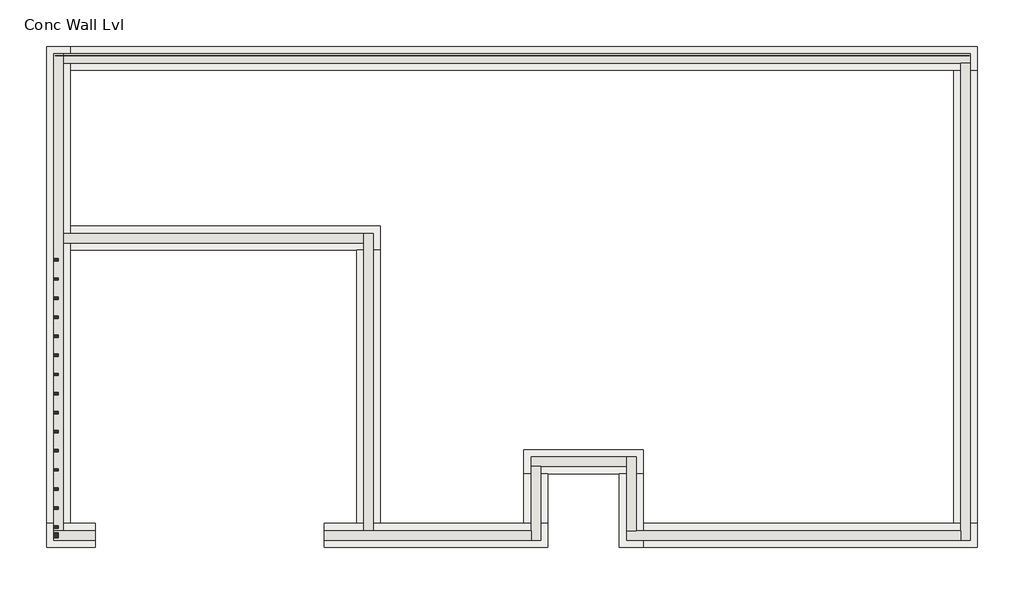
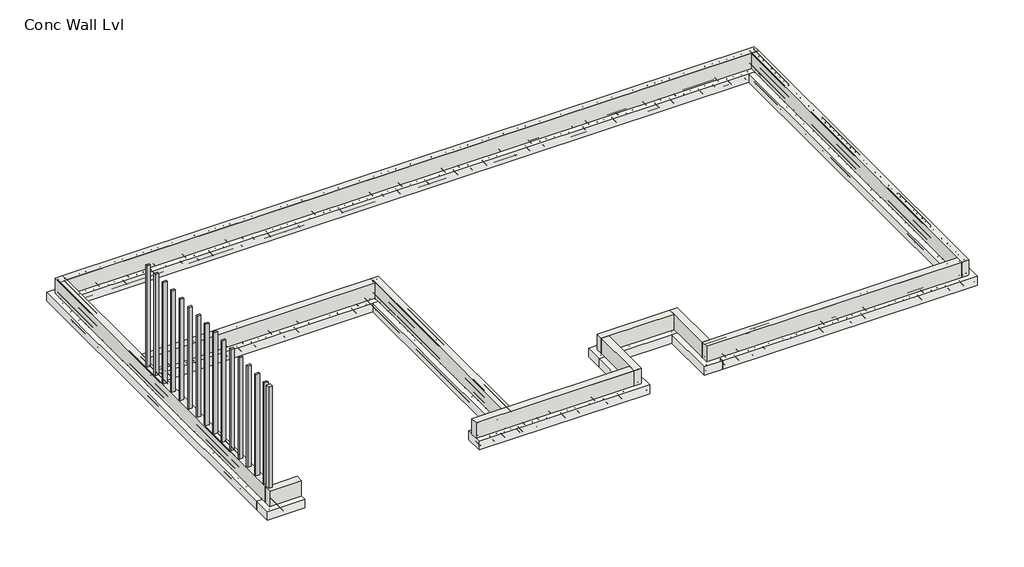
# One storey, part 1 of 4: 16 columns, 11 footings, 11 walls.
"""IFC4 building model written with IfcOpenShell, lengths in millimetres."""

import ifcopenshell
import ifcopenshell.guid

model = None  # the IFC model being written
_history = None  # IfcOwnerHistory: only IFC2X3 demands one
_inside = {}  # id of a spatial element -> (the spatial element, [elements in it])
_under = {}  # id of a project, library or spatial element -> (it, [spatial elements below it])
_declared = {}  # id of a project -> (the project, [libraries it declares])
_typed = {}  # id of a type object -> (the type object, [elements of that type])
_made_of = {}  # id of a material, layer set ... -> (it, [elements and type objects made of it])


def new_model(schema):
    """Start an empty IFC model of exactly this schema.

    Asked for "IFC4X3", IfcOpenShell would pick the latest addendum, in which some entities
    have other attributes; the version numbers below select the first issue.
    IFC2X3 requires an IfcOwnerHistory on every rooted entity: one is made here for all.
    """
    global model, _history
    if schema == "IFC4X3":
        model = ifcopenshell.file(schema_version=(4, 3, 0, 0))
    else:
        model = ifcopenshell.file(schema=schema)
    _inside.clear()
    _under.clear()
    _declared.clear()
    _typed.clear()
    _made_of.clear()
    _history = None
    if model.schema == "IFC2X3":
        org = make("IfcOrganization", Name="unknown")
        user = make(
            "IfcPersonAndOrganization",
            ThePerson=make("IfcPerson", FamilyName="unknown"),
            TheOrganization=org,
        )
        app = make(
            "IfcApplication",
            ApplicationDeveloper=org,
            Version="unknown",
            ApplicationFullName="unknown",
            ApplicationIdentifier="unknown",
        )
        _history = make(
            "IfcOwnerHistory",
            OwningUser=user,
            OwningApplication=app,
            ChangeAction="ADDED",
            CreationDate=0,
        )
    return model


def make(cls, **values):
    """One entity of the class cls with the attributes given. An attribute that is None is left unset."""
    return model.create_entity(
        cls, **{name: value for name, value in values.items() if value is not None}
    )


def rooted(cls, **values):
    """An entity with a GlobalId (a new one), such as an element, a storey or a relation."""
    return make(cls, GlobalId=ifcopenshell.guid.new(), OwnerHistory=_history, **values)


def si_unit(unit_type, name, prefix=None):
    """IfcSIUnit, for example si_unit("LENGTHUNIT", "METRE", prefix="MILLI")."""
    return make("IfcSIUnit", UnitType=unit_type, Prefix=prefix, Name=name)


def assignment(units):
    """IfcUnitAssignment: the units of a project."""
    return None if units is None else make("IfcUnitAssignment", Units=units)


def point(xyz):
    """IfcCartesianPoint."""
    return None if xyz is None else make("IfcCartesianPoint", Coordinates=xyz)


def direction(xyz):
    """IfcDirection."""
    return None if xyz is None else make("IfcDirection", DirectionRatios=xyz)


def frame(location, z_axis=None, x_axis=None):
    """IfcAxis2Placement3D, a coordinate frame: its origin and axes. An axis left out is left unset."""
    return make(
        "IfcAxis2Placement3D",
        Location=point(location),
        Axis=direction(z_axis),
        RefDirection=direction(x_axis),
    )


def origin():
    """The frame at (0, 0, 0) with its axes left unset."""
    return frame((0.0, 0.0, 0.0))


def place(relative_to, where):
    """IfcLocalPlacement: puts the frame where relative to a parent placement (None: the world)."""
    return make(
        "IfcLocalPlacement", PlacementRelTo=relative_to, RelativePlacement=where
    )


def context(
    kind, dimensions, precision=None, world=None, true_north=None, identifier=None
):
    """IfcGeometricRepresentationContext, for example the 3D "Model" context."""
    return make(
        "IfcGeometricRepresentationContext",
        ContextIdentifier=identifier,
        ContextType=kind,
        CoordinateSpaceDimension=dimensions,
        Precision=precision,
        WorldCoordinateSystem=world,
        TrueNorth=true_north,
    )


def project(units=None, contexts=None):
    """IfcProject with its units and contexts."""
    return rooted(
        "IfcProject",
        Name="project",
        RepresentationContexts=contexts,
        UnitsInContext=assignment(units),
    )


def spatial(cls, under=None, at=None, **own):
    """A site, building, storey or space (cls), placed at a placement, below another one or the project."""
    s = rooted(cls, ObjectPlacement=at, **own)
    if under is not None:
        _under.setdefault(under.id(), (under, []))[1].append(s)
    return s


def polyline(points):
    """IfcPolyline through the points."""
    return make("IfcPolyline", Points=[point(p) for p in points])


def outline(outer, holes=None, kind="AREA"):
    """IfcArbitraryClosedProfileDef: a profile drawn as a closed curve; with holes, ...WithVoids."""
    if holes is None:
        return make("IfcArbitraryClosedProfileDef", ProfileType=kind, OuterCurve=outer)
    return make(
        "IfcArbitraryProfileDefWithVoids",
        ProfileType=kind,
        OuterCurve=outer,
        InnerCurves=holes,
    )


def extrude(swept, where, along, depth):
    """IfcExtrudedAreaSolid: the profile swept, set in the frame where, extruded along a direction by depth."""
    return make(
        "IfcExtrudedAreaSolid",
        SweptArea=swept,
        Position=where,
        ExtrudedDirection=direction(along),
        Depth=depth,
    )


def faces_of(points, faces, orient=None, outer=None):
    """IfcFace entities. A face is a list of loops; a loop is a list of indices into points, from 0.

    orient and outer hold one flag for each loop. By default every Orientation is true, the
    first loop of a face is its IfcFaceOuterBound and the others are IfcFaceBound.
    """
    made = []
    for i, loops in enumerate(faces):
        bounds = []
        for j, loop in enumerate(loops):
            is_outer = j == 0 if outer is None else outer[i][j]
            bounds.append(
                make(
                    "IfcFaceOuterBound" if is_outer else "IfcFaceBound",
                    Bound=make("IfcPolyLoop", Polygon=[points[k] for k in loop]),
                    Orientation=True if orient is None else orient[i][j],
                )
            )
        made.append(make("IfcFace", Bounds=bounds))
    return made


def faceted_brep(points, faces, orient=None, outer=None, voids=None):
    """IfcFacetedBrep: a solid bounded by flat faces; with voids (closed shells), ...WithVoids."""
    shared = [point(p) for p in points]
    hull = make("IfcClosedShell", CfsFaces=faces_of(shared, faces, orient, outer))
    if voids is None:
        return make("IfcFacetedBrep", Outer=hull)
    return make(
        "IfcFacetedBrepWithVoids",
        Outer=hull,
        Voids=[
            make(cls, CfsFaces=faces_of(shared, fs, o, b)) for cls, fs, o, b in voids
        ],
    )


def shape(context_of_items, identifier, shape_type, items):
    """IfcShapeRepresentation: the items that make up one representation, for example the "Body"."""
    return make(
        "IfcShapeRepresentation",
        ContextOfItems=context_of_items,
        RepresentationIdentifier=identifier,
        RepresentationType=shape_type,
        Items=items,
    )


def source(mapping_origin, context_of_items, identifier, shape_type, items):
    """IfcRepresentationMap: a shape defined once, which mapped items show again and again."""
    return make(
        "IfcRepresentationMap",
        MappingOrigin=mapping_origin,
        MappedRepresentation=shape(context_of_items, identifier, shape_type, items),
    )


def transform(
    local_origin,
    x_axis=None,
    y_axis=None,
    z_axis=None,
    scale=None,
    scale2=None,
    scale3=None,
    uniform=True,
):
    """IfcCartesianTransformationOperator3D, or its non-uniform kind. x_axis, y_axis, z_axis: its Axis1, 2, 3."""
    if uniform:
        return make(
            "IfcCartesianTransformationOperator3D",
            Axis1=direction(x_axis),
            Axis2=direction(y_axis),
            LocalOrigin=point(local_origin),
            Scale=scale,
            Axis3=direction(z_axis),
        )
    return make(
        "IfcCartesianTransformationOperator3DnonUniform",
        Axis1=direction(x_axis),
        Axis2=direction(y_axis),
        LocalOrigin=point(local_origin),
        Scale=scale,
        Axis3=direction(z_axis),
        Scale2=scale2,
        Scale3=scale3,
    )


def mapped(mapping_source, mapping_target):
    """IfcMappedItem: shows the shape of a source again, moved by a transform."""
    return make(
        "IfcMappedItem", MappingSource=mapping_source, MappingTarget=mapping_target
    )


def made_of(thing, what):
    """Note that an element or type object is made of a material, layer set ...; save() writes the relation."""
    if what is not None:
        _made_of.setdefault(what.id(), (what, []))[1].append(thing)
    return thing


def element(
    cls,
    number,
    at=None,
    inside=None,
    cuts=None,
    type_object=None,
    material=None,
    context=None,
    identifier="Body",
    shape_type=None,
    held_by="IfcProductDefinitionShape",
    body=None,
    shapes=None,
    **own,
):
    """One element of the class cls, such as IfcWall. Its Tag is "e" and its number.

    at: its placement. inside: the storey or other place that contains it. cuts: it is an
    opening in that element (IfcRelVoidsElement). A single representation is given by context,
    identifier, shape_type and body (its items); several are given by shapes. held_by: the class
    of the entity that holds the representations. save() writes the other relations.
    """
    e = rooted(cls, Tag="e%d" % number, ObjectPlacement=at, **own)
    if body is not None:
        shapes = [shape(context, identifier, shape_type, body)]
    if shapes is not None:
        e.Representation = make(held_by, Representations=shapes)
    if inside is not None:
        _inside.setdefault(inside.id(), (inside, []))[1].append(e)
    if cuts is not None:
        rooted(
            "IfcRelVoidsElement", RelatingBuildingElement=cuts, RelatedOpeningElement=e
        )
    if type_object is not None:
        _typed.setdefault(type_object.id(), (type_object, []))[1].append(e)
    return made_of(e, material)


def aggregate(whole, parts):
    """IfcRelAggregates: a whole, such as a stair, and the parts it consists of."""
    return rooted("IfcRelAggregates", RelatingObject=whole, RelatedObjects=parts)


def save(model, path):
    """Write the relations noted so far, then the file.

    IfcRelAggregates (storeys below a building ...), IfcRelContainedInSpatialStructure (elements
    in a storey), IfcRelDefinesByType, IfcRelAssociatesMaterial and IfcRelDeclares: one each for
    every whole, place, type object, material and project.
    """
    for whole, parts in _under.values():
        aggregate(whole, parts)
    for where, things in _inside.values():
        rooted(
            "IfcRelContainedInSpatialStructure",
            RelatedElements=things,
            RelatingStructure=where,
        )
    for kind, things in _typed.values():
        rooted("IfcRelDefinesByType", RelatedObjects=things, RelatingType=kind)
    for what, things in _made_of.values():
        rooted("IfcRelAssociatesMaterial", RelatedObjects=things, RelatingMaterial=what)
    for by, libraries in _declared.values():
        rooted("IfcRelDeclares", RelatingContext=by, RelatedDefinitions=libraries)
    model.write(path)


def timber_column_4ee0a357(model_context):
    return source(origin(), model_context, "Body", "SweptSolid", [
        extrude(outline(polyline([(25.4, 50.8), (25.4, -50.8), (-25.4, -50.8), (-25.4, 50.8), (25.4, 50.8)])), frame((0.0, 0.0, -319.88125), z_axis=(0.0, 0.0, 1.0), x_axis=(1.0, 0.0, 0.0)), (0.0, 0.0, 1.0), 2986.88125),
    ])


def timber_column_8a3ad47c(model_context):
    return source(origin(), model_context, "Body", "SweptSolid", [
        extrude(outline(polyline([(50.8, 50.8), (50.8, -50.8), (-50.8, -50.8), (-50.8, 50.8), (50.8, 50.8)])), frame((0.0, 0.0, -319.88125), z_axis=(0.0, 0.0, 1.0), x_axis=(1.0, 0.0, 0.0)), (0.0, 0.0, 1.0), 2986.88125),
    ])


model = new_model("IFC4")

# Units and contexts
model_context = context("Model", 3, world=origin())
ifc_project = project(units=[si_unit("LENGTHUNIT", "METRE", prefix="MILLI")], contexts=[model_context])

# Site, building, storey
site = spatial("IfcSite", under=ifc_project)
building = spatial("IfcBuilding", under=site)
storey = spatial("IfcBuildingStorey", under=building, Name="Conc Wall Lvl", Elevation=-370.68125)

# Columns
placement = place(None, origin())
timber_column_shape = timber_column_4ee0a357(model_context)
element("IfcColumn", 1, ObjectType="Timber-Column : BLDG 6241 Wall Struds 2\"x4\"", at=placement, inside=storey, context=model_context, shape_type="MappedRepresentation", body=[
    mapped(timber_column_shape, transform((-17750.414829, 813.5284114, 0.0), x_axis=(0.0, 1.0, 0.0), y_axis=(-1.0, 0.0, 0.0), z_axis=(0.0, 0.0, 1.0))),
])
element("IfcColumn", 2, ObjectType="Timber-Column : BLDG 6241 Wall Struds 2\"x4\"", at=placement, inside=storey, context=model_context, shape_type="MappedRepresentation", body=[
    mapped(timber_column_shape, transform((-17750.414829, 407.1284114, 0.0), x_axis=(0.0, 1.0, 0.0), y_axis=(-1.0, 0.0, 0.0), z_axis=(0.0, 0.0, 1.0))),
])
element("IfcColumn", 3, ObjectType="Timber-Column : BLDG 6241 Wall Struds 2\"x4\"", at=placement, inside=storey, context=model_context, shape_type="MappedRepresentation", body=[
    mapped(timber_column_shape, transform((-17750.414829, 0.7284114, 0.0), x_axis=(0.0, 1.0, 0.0), y_axis=(-1.0, 0.0, 0.0), z_axis=(0.0, 0.0, 1.0))),
])
element("IfcColumn", 4, ObjectType="Timber-Column : BLDG 6241 Wall Struds 2\"x4\"", at=placement, inside=storey, context=model_context, shape_type="MappedRepresentation", body=[
    mapped(timber_column_shape, transform((-17750.414829, -405.6715886, 0.0), x_axis=(0.0, 1.0, 0.0), y_axis=(-1.0, 0.0, 0.0), z_axis=(0.0, 0.0, 1.0))),
])
element("IfcColumn", 5, ObjectType="Timber-Column : BLDG 6241 Wall Struds 2\"x4\"", at=placement, inside=storey, context=model_context, shape_type="MappedRepresentation", body=[
    mapped(timber_column_shape, transform((-17750.414829, -812.0715886, 0.0), x_axis=(0.0, 1.0, 0.0), y_axis=(-1.0, 0.0, 0.0), z_axis=(0.0, 0.0, 1.0))),
])
element("IfcColumn", 6, ObjectType="Timber-Column : BLDG 6241 Wall Struds 2\"x4\"", at=placement, inside=storey, context=model_context, shape_type="MappedRepresentation", body=[
    mapped(timber_column_shape, transform((-17750.414829, -1218.4715886, 0.0), x_axis=(0.0, 1.0, 0.0), y_axis=(-1.0, 0.0, 0.0), z_axis=(0.0, 0.0, 1.0))),
])
element("IfcColumn", 7, ObjectType="Timber-Column : BLDG 6241 Wall Struds 2\"x4\"", at=placement, inside=storey, context=model_context, shape_type="MappedRepresentation", body=[
    mapped(timber_column_shape, transform((-17750.414829, -1624.8715886, 0.0), x_axis=(0.0, 1.0, 0.0), y_axis=(-1.0, 0.0, 0.0), z_axis=(0.0, 0.0, 1.0))),
])
element("IfcColumn", 8, ObjectType="Timber-Column : BLDG 6241 Wall Struds 2\"x4\"", at=placement, inside=storey, context=model_context, shape_type="MappedRepresentation", body=[
    mapped(timber_column_shape, transform((-17750.414829, -2031.2715886, 0.0), x_axis=(0.0, 1.0, 0.0), y_axis=(-1.0, 0.0, 0.0), z_axis=(0.0, 0.0, 1.0))),
])
element("IfcColumn", 9, ObjectType="Timber-Column : BLDG 6241 Wall Struds 2\"x4\"", at=placement, inside=storey, context=model_context, shape_type="MappedRepresentation", body=[
    mapped(timber_column_shape, transform((-17750.414829, -2437.6715886, 0.0), x_axis=(0.0, 1.0, 0.0), y_axis=(-1.0, 0.0, 0.0), z_axis=(0.0, 0.0, 1.0))),
])
element("IfcColumn", 10, ObjectType="Timber-Column : BLDG 6241 Wall Struds 2\"x4\"", at=placement, inside=storey, context=model_context, shape_type="MappedRepresentation", body=[
    mapped(timber_column_shape, transform((-17750.414829, -2844.0715886, 0.0), x_axis=(0.0, 1.0, 0.0), y_axis=(-1.0, 0.0, 0.0), z_axis=(0.0, 0.0, 1.0))),
])
element("IfcColumn", 11, ObjectType="Timber-Column : BLDG 6241 Wall Struds 2\"x4\"", at=placement, inside=storey, context=model_context, shape_type="MappedRepresentation", body=[
    mapped(timber_column_shape, transform((-17750.414829, -3250.4715886, 0.0), x_axis=(0.0, 1.0, 0.0), y_axis=(-1.0, 0.0, 0.0), z_axis=(0.0, 0.0, 1.0))),
])
element("IfcColumn", 12, ObjectType="Timber-Column : BLDG 6241 Wall Struds 2\"x4\"", at=placement, inside=storey, context=model_context, shape_type="MappedRepresentation", body=[
    mapped(timber_column_shape, transform((-17750.414829, -3656.8715886, 0.0), x_axis=(0.0, 1.0, 0.0), y_axis=(-1.0, 0.0, 0.0), z_axis=(0.0, 0.0, 1.0))),
])
element("IfcColumn", 13, ObjectType="Timber-Column : BLDG 6241 Wall Struds 2\"x4\"", at=placement, inside=storey, context=model_context, shape_type="MappedRepresentation", body=[
    mapped(timber_column_shape, transform((-17750.414829, -4063.2715886, 0.0), x_axis=(0.0, 1.0, 0.0), y_axis=(-1.0, 0.0, 0.0), z_axis=(0.0, 0.0, 1.0))),
])
element("IfcColumn", 14, ObjectType="Timber-Column : BLDG 6241 Wall Struds 2\"x4\"", at=placement, inside=storey, context=model_context, shape_type="MappedRepresentation", body=[
    mapped(timber_column_shape, transform((-17750.414829, -4469.6715886, 0.0), x_axis=(0.0, 1.0, 0.0), y_axis=(-1.0, 0.0, 0.0), z_axis=(0.0, 0.0, 1.0))),
])
element("IfcColumn", 15, ObjectType="Timber-Column : BLDG 6241 Wall Struds 2\"x4\"", at=placement, inside=storey, context=model_context, shape_type="MappedRepresentation", body=[
    mapped(timber_column_shape, transform((-17750.414829, -4876.0715886, 0.0), x_axis=(0.0, 1.0, 0.0), y_axis=(-1.0, 0.0, 0.0), z_axis=(0.0, 0.0, 1.0))),
])
timber_column_2_shape = timber_column_8a3ad47c(model_context)
element("IfcColumn", 16, ObjectType="Timber-Column : BLDG 6241 Wall Struds 4\"x4\"", at=placement, inside=storey, context=model_context, shape_type="MappedRepresentation", body=[
    mapped(timber_column_2_shape, transform((-17750.414829, -5053.8715886, 0.0), x_axis=(1.0, 0.0, 0.0), y_axis=(0.0, 1.0, 0.0), z_axis=(0.0, 0.0, 1.0))),
])

# Footings
element("IfcFooting", 17, ObjectType="BLDG Conc Footing - 20\" x 10\"", at=placement, inside=storey, context=model_context, shape_type="Brep", body=[
    faceted_brep([(-16915.389829, -4799.8715886, -827.88125), (-16915.389829, -5307.8715886, -827.88125), (-16915.389829, -5307.8715886, -1081.88125), (-16915.389829, -4799.8715886, -1081.88125), (-17445.614829, -4799.8715886, -827.88125), (-17953.614829, -4799.8715886, -827.88125), (-17953.614829, -5307.8715886, -827.88125), (-17953.614829, -5307.8715886, -1081.88125), (-17953.614829, -4799.8715886, -1081.88125), (-17445.614829, -4799.8715886, -1081.88125)], [[[0, 1, 2, 3]], [[0, 4, 5, 6, 1]], [[2, 1, 6, 7]], [[3, 2, 7, 8, 9]], [[0, 3, 9, 8, 5, 4]], [[6, 5, 8, 7]]]),
])
element("IfcFooting", 18, ObjectType="BLDG Conc Footing - 20\" x 10\"", at=placement, inside=storey, context=model_context, shape_type="Brep", body=[
    faceted_brep([(-17445.614829, 5360.1284114, -827.88125), (-17953.614829, 5360.1284114, -827.88125), (-17953.614829, -4799.8715886, -827.88125), (-17445.614829, -4799.8715886, -827.88125), (-17445.614829, 1023.0784114, -827.88125), (-17445.614829, 1531.0784114, -827.88125), (-17445.614829, 4852.1284114, -827.88125), (-17953.614829, 5360.1284114, -1081.88125), (-17953.614829, -4799.8715886, -1081.88125), (-17445.614829, 5360.1284114, -1081.88125), (-17445.614829, 4852.1284114, -1081.88125), (-17445.614829, 1531.0784114, -1081.88125), (-17445.614829, 1023.0784114, -1081.88125), (-17445.614829, -4799.8715886, -1081.88125)], [[[0, 1, 2, 3, 4, 5, 6]], [[1, 7, 8, 2]], [[7, 9, 10, 11, 12, 13, 8]], [[9, 0, 6, 5, 4, 3, 13, 12, 11, 10]], [[3, 2, 8, 13]], [[1, 0, 9, 7]]]),
])
element("IfcFooting", 19, ObjectType="BLDG Conc Footing - 20\" x 10\"", at=placement, inside=storey, context=model_context, shape_type="Brep", body=[
    faceted_brep([(-10847.964829, 1531.0784114, -827.88125), (-17445.614829, 1531.0784114, -827.88125), (-17445.614829, 1023.0784114, -827.88125), (-11355.964829, 1023.0784114, -827.88125), (-10847.964829, 1023.0784114, -827.88125), (-10847.964829, 1023.0784114, -1081.88125), (-17445.614829, 1023.0784114, -1081.88125), (-11355.964829, 1023.0784114, -1081.88125), (-10847.964829, 1531.0784114, -1081.88125), (-17445.614829, 1531.0784114, -1081.88125)], [[[0, 1, 2, 3, 4]], [[5, 4, 3, 2, 6, 7]], [[8, 5, 7, 6, 9]], [[0, 8, 9, 1]], [[2, 1, 9, 6]], [[0, 4, 5, 8]]]),
])
element("IfcFooting", 20, ObjectType="BLDG Conc Footing - 20\" x 10\"", at=placement, inside=storey, context=model_context, shape_type="SweptSolid", body=[
    extrude(outline(polyline([(-10847.964829, -4799.8715886), (-11355.964829, -4799.8715886), (-11355.964829, 1023.0784114), (-10847.964829, 1023.0784114), (-10847.964829, -4799.8715886)])), frame((0.0, 0.0, -1081.88125), z_axis=(0.0, 0.0, 1.0), x_axis=(1.0, 0.0, 0.0)), (0.0, 0.0, 1.0), 254.0),
])
element("IfcFooting", 21, ObjectType="BLDG Conc Footing - 20\" x 10\"", at=placement, inside=storey, context=model_context, shape_type="Brep", body=[
    faceted_brep([(-12038.589829, -5307.8715886, -827.88125), (-12038.589829, -4799.8715886, -827.88125), (-12038.589829, -4799.8715886, -1081.88125), (-12038.589829, -5307.8715886, -1081.88125), (-7285.614829, -4799.8715886, -827.88125), (-7793.614829, -4799.8715886, -827.88125), (-10847.964829, -4799.8715886, -827.88125), (-11355.964829, -4799.8715886, -827.88125), (-7285.614829, -5307.8715886, -827.88125), (-7285.614829, -5307.8715886, -1081.88125), (-7285.614829, -4799.8715886, -1081.88125), (-11355.964829, -4799.8715886, -1081.88125), (-10847.964829, -4799.8715886, -1081.88125), (-7793.614829, -4799.8715886, -1081.88125)], [[[0, 1, 2, 3]], [[4, 5, 6, 7, 1, 0, 8]], [[9, 8, 0, 3]], [[10, 9, 3, 2, 11, 12, 13]], [[4, 10, 13, 12, 11, 2, 1, 7, 6, 5]], [[4, 8, 9, 10]]]),
])
element("IfcFooting", 22, ObjectType="BLDG Conc Footing - 20\" x 10\"", at=placement, inside=storey, context=model_context, shape_type="Brep", body=[
    faceted_brep([(-5253.614829, -3231.4215886, -827.88125), (-7793.614829, -3231.4215886, -827.88125), (-7793.614829, -3739.4215886, -827.88125), (-7285.614829, -3739.4215886, -827.88125), (-5761.614829, -3739.4215886, -827.88125), (-5253.614829, -3739.4215886, -827.88125), (-5253.614829, -3739.4215886, -1081.88125), (-7793.614829, -3739.4215886, -1081.88125), (-7285.614829, -3739.4215886, -1081.88125), (-5761.614829, -3739.4215886, -1081.88125), (-5253.614829, -3231.4215886, -1081.88125), (-7793.614829, -3231.4215886, -1081.88125)], [[[0, 1, 2, 3, 4, 5]], [[6, 5, 4, 3, 2, 7, 8, 9]], [[10, 6, 9, 8, 7, 11]], [[0, 10, 11, 1]], [[0, 5, 6, 10]], [[2, 1, 11, 7]]]),
])
element("IfcFooting", 23, ObjectType="BLDG Conc Footing - 20\" x 10\"", at=placement, inside=storey, context=model_context, shape_type="Brep", body=[
    faceted_brep([(-5761.614829, -5307.8715886, -827.88125), (-5253.614829, -5307.8715886, -827.88125), (-5253.614829, -4799.8715886, -827.88125), (-5253.614829, -3739.4215886, -827.88125), (-5761.614829, -3739.4215886, -827.88125), (-5761.614829, -5307.8715886, -1081.88125), (-5761.614829, -3739.4215886, -1081.88125), (-5253.614829, -5307.8715886, -1081.88125), (-5253.614829, -3739.4215886, -1081.88125), (-5253.614829, -4799.8715886, -1081.88125)], [[[0, 1, 2, 3, 4]], [[5, 0, 4, 6]], [[7, 5, 6, 8, 9]], [[1, 7, 9, 8, 3, 2]], [[4, 3, 8, 6]], [[1, 0, 5, 7]]]),
])
element("IfcFooting", 24, ObjectType="BLDG Conc Footing - 20\" x 10\"", at=placement, inside=storey, context=model_context, shape_type="Brep", body=[
    faceted_brep([(1858.385171, -5307.8715886, -827.88125), (1858.385171, -4799.8715886, -827.88125), (1350.385171, -4799.8715886, -827.88125), (-5253.614829, -4799.8715886, -827.88125), (-5253.614829, -5307.8715886, -827.88125), (1858.385171, -5307.8715886, -1081.88125), (-5253.614829, -5307.8715886, -1081.88125), (1858.385171, -4799.8715886, -1081.88125), (-5253.614829, -4799.8715886, -1081.88125), (1350.385171, -4799.8715886, -1081.88125)], [[[0, 1, 2, 3, 4]], [[5, 0, 4, 6]], [[7, 5, 6, 8, 9]], [[1, 7, 9, 8, 3, 2]], [[4, 3, 8, 6]], [[1, 0, 5, 7]]]),
])
element("IfcFooting", 25, ObjectType="BLDG Conc Footing - 20\" x 10\"", at=placement, inside=storey, context=model_context, shape_type="SweptSolid", body=[
    extrude(outline(polyline([(-7285.614829, -4799.8715886), (-7793.614829, -4799.8715886), (-7793.614829, -3739.4215886), (-7285.614829, -3739.4215886), (-7285.614829, -4799.8715886)])), frame((0.0, 0.0, -1081.88125), z_axis=(0.0, 0.0, 1.0), x_axis=(1.0, 0.0, 0.0)), (0.0, 0.0, 1.0), 254.0),
])
element("IfcFooting", 26, ObjectType="BLDG Conc Footing - 20\" x 10\"", at=placement, inside=storey, context=model_context, shape_type="Brep", body=[
    faceted_brep([(1858.385171, 4852.1284114, -827.88125), (1858.385171, 5360.1284114, -827.88125), (-17445.614829, 5360.1284114, -827.88125), (-17445.614829, 4852.1284114, -827.88125), (1350.385171, 4852.1284114, -827.88125), (1858.385171, 5360.1284114, -1081.88125), (-17445.614829, 5360.1284114, -1081.88125), (1858.385171, 4852.1284114, -1081.88125), (1350.385171, 4852.1284114, -1081.88125), (-17445.614829, 4852.1284114, -1081.88125)], [[[0, 1, 2, 3, 4]], [[1, 5, 6, 2]], [[5, 7, 8, 9, 6]], [[7, 0, 4, 3, 9, 8]], [[3, 2, 6, 9]], [[1, 0, 7, 5]]]),
])
element("IfcFooting", 27, ObjectType="BLDG Conc Footing - 20\" x 10\"", at=placement, inside=storey, context=model_context, shape_type="SweptSolid", body=[
    extrude(outline(polyline([(1858.385171, -4799.8715886), (1350.385171, -4799.8715886), (1350.385171, 4852.1284114), (1858.385171, 4852.1284114), (1858.385171, -4799.8715886)])), frame((0.0, 0.0, -1081.88125), z_axis=(0.0, 0.0, 1.0), x_axis=(1.0, 0.0, 0.0)), (0.0, 0.0, 1.0), 254.0),
])

# Walls
element("IfcWall", 28, ObjectType="BLDG 6241 Conc Wall - 8\"", at=placement, inside=storey, context=model_context, shape_type="Brep", body=[
    faceted_brep([(-16915.389829, -4952.2715886, -827.88125), (-17598.014829, -4952.2715886, -827.88125), (-17801.214829, -4952.2715886, -827.88125), (-17801.214829, -4952.2715886, -370.68125), (-17598.014829, -4952.2715886, -370.68125), (-16915.389829, -4952.2715886, -370.68125), (-16915.389829, -5155.4715886, -827.88125), (-16915.389829, -5155.4715886, -370.68125), (-17801.214829, -5155.4715886, -370.68125), (-17801.214829, -5155.4715886, -827.88125)], [[[0, 1, 2, 3, 4, 5]], [[6, 7, 8, 9]], [[2, 1, 0, 6, 9]], [[5, 4, 3, 8, 7]], [[0, 5, 7, 6]], [[3, 2, 9, 8]]]),
])
element("IfcWall", 29, ObjectType="BLDG 6241 Conc Wall - 8\"", at=placement, inside=storey, context=model_context, shape_type="Brep", body=[
    faceted_brep([(-17598.014829, -4952.2715886, -827.88125), (-17598.014829, 1175.4784114, -827.88125), (-17598.014829, 1378.6784114, -827.88125), (-17598.014829, 5004.5284114, -827.88125), (-17598.014829, 5207.7284114, -827.88125), (-17598.014829, 5207.7284114, -370.68125), (-17598.014829, 5004.5284114, -370.68125), (-17598.014829, 1378.6784114, -370.68125), (-17598.014829, 1175.4784114, -370.68125), (-17598.014829, -4952.2715886, -370.68125), (-17801.214829, -4952.2715886, -827.88125), (-17801.214829, -4952.2715886, -370.68125), (-17801.214829, 5207.7284114, -370.68125), (-17801.214829, 5207.7284114, -827.88125)], [[[0, 1, 2, 3, 4, 5, 6, 7, 8, 9]], [[10, 11, 12, 13]], [[4, 3, 2, 1, 0, 10, 13]], [[9, 8, 7, 6, 5, 12, 11]], [[0, 9, 11, 10]], [[5, 4, 13, 12]]]),
])
element("IfcWall", 30, ObjectType="BLDG 6241 Conc Wall - 8\"", at=placement, inside=storey, context=model_context, shape_type="Brep", body=[
    faceted_brep([(-17598.014829, 5004.5284114, -827.88125), (1502.785171, 5004.5284114, -827.88125), (1705.985171, 5004.5284114, -827.88125), (1705.985171, 5004.5284114, -370.68125), (1502.785171, 5004.5284114, -370.68125), (-17598.014829, 5004.5284114, -370.68125), (-17598.014829, 5207.7284114, -827.88125), (-17598.014829, 5207.7284114, -370.68125), (1705.985171, 5207.7284114, -370.68125), (1705.985171, 5207.7284114, -827.88125)], [[[0, 1, 2, 3, 4, 5]], [[6, 7, 8, 9]], [[2, 1, 0, 6, 9]], [[5, 4, 3, 8, 7]], [[0, 5, 7, 6]], [[3, 2, 9, 8]]]),
])
element("IfcWall", 31, ObjectType="BLDG 6241 Conc Wall - 8\"", at=placement, inside=storey, context=model_context, shape_type="Brep", body=[
    faceted_brep([(1502.785171, 5004.5284114, -827.88125), (1502.785171, -4952.2715886, -827.88125), (1502.785171, -5155.4715886, -827.88125), (1502.785171, -5155.4715886, -370.68125), (1502.785171, -4952.2715886, -370.68125), (1502.785171, 5004.5284114, -370.68125), (1705.985171, 5004.5284114, -827.88125), (1705.985171, 5004.5284114, -370.68125), (1705.985171, -5155.4715886, -370.68125), (1705.985171, -5155.4715886, -827.88125)], [[[0, 1, 2, 3, 4, 5]], [[6, 7, 8, 9]], [[2, 1, 0, 6, 9]], [[5, 4, 3, 8, 7]], [[0, 5, 7, 6]], [[3, 2, 9, 8]]]),
])
element("IfcWall", 32, ObjectType="BLDG 6241 Conc Wall - 8\"", at=placement, inside=storey, context=model_context, shape_type="Brep", body=[
    faceted_brep([(1502.785171, -4952.2715886, -827.88125), (-5406.014829, -4952.2715886, -827.88125), (-5609.214829, -4952.2715886, -827.88125), (-5609.214829, -4952.2715886, -370.68125), (-5406.014829, -4952.2715886, -370.68125), (1502.785171, -4952.2715886, -370.68125), (1502.785171, -5155.4715886, -827.88125), (1502.785171, -5155.4715886, -370.68125), (-5609.214829, -5155.4715886, -370.68125), (-5609.214829, -5155.4715886, -827.88125)], [[[0, 1, 2, 3, 4, 5]], [[6, 7, 8, 9]], [[2, 1, 0, 6, 9]], [[5, 4, 3, 8, 7]], [[0, 5, 7, 6]], [[3, 2, 9, 8]]]),
])
element("IfcWall", 33, ObjectType="BLDG 6241 Conc Wall - 8\"", at=placement, inside=storey, context=model_context, shape_type="Brep", body=[
    faceted_brep([(-5406.014829, -4952.2715886, -827.88125), (-5406.014829, -3383.8215886, -827.88125), (-5406.014829, -3383.8215886, -370.68125), (-5406.014829, -4952.2715886, -370.68125), (-5609.214829, -4952.2715886, -827.88125), (-5609.214829, -4952.2715886, -370.68125), (-5609.214829, -3587.0215886, -370.68125), (-5609.214829, -3383.8215886, -370.68125), (-5609.214829, -3383.8215886, -827.88125), (-5609.214829, -3587.0215886, -827.88125)], [[[0, 1, 2, 3]], [[4, 5, 6, 7, 8, 9]], [[1, 0, 4, 9, 8]], [[3, 2, 7, 6, 5]], [[0, 3, 5, 4]], [[2, 1, 8, 7]]]),
])
element("IfcWall", 34, ObjectType="BLDG 6241 Conc Wall - 8\"", at=placement, inside=storey, context=model_context, shape_type="Brep", body=[
    faceted_brep([(-5609.214829, -3383.8215886, -827.88125), (-7641.214829, -3383.8215886, -827.88125), (-7641.214829, -3383.8215886, -370.68125), (-5609.214829, -3383.8215886, -370.68125), (-5609.214829, -3587.0215886, -827.88125), (-5609.214829, -3587.0215886, -370.68125), (-7438.014829, -3587.0215886, -370.68125), (-7641.214829, -3587.0215886, -370.68125), (-7641.214829, -3587.0215886, -827.88125), (-7438.014829, -3587.0215886, -827.88125)], [[[0, 1, 2, 3]], [[4, 5, 6, 7, 8, 9]], [[1, 0, 4, 9, 8]], [[3, 2, 7, 6, 5]], [[0, 3, 5, 4]], [[2, 1, 8, 7]]]),
])
element("IfcWall", 35, ObjectType="BLDG 6241 Conc Wall - 8\"", at=placement, inside=storey, context=model_context, shape_type="Brep", body=[
    faceted_brep([(-7641.214829, -3587.0215886, -827.88125), (-7641.214829, -4952.2715886, -827.88125), (-7641.214829, -5155.4715886, -827.88125), (-7641.214829, -5155.4715886, -370.68125), (-7641.214829, -4952.2715886, -370.68125), (-7641.214829, -3587.0215886, -370.68125), (-7438.014829, -3587.0215886, -827.88125), (-7438.014829, -3587.0215886, -370.68125), (-7438.014829, -5155.4715886, -370.68125), (-7438.014829, -5155.4715886, -827.88125)], [[[0, 1, 2, 3, 4, 5]], [[6, 7, 8, 9]], [[2, 1, 0, 6, 9]], [[5, 4, 3, 8, 7]], [[0, 5, 7, 6]], [[3, 2, 9, 8]]]),
])
element("IfcWall", 36, ObjectType="BLDG 6241 Conc Wall - 8\"", at=placement, inside=storey, context=model_context, shape_type="Brep", body=[
    faceted_brep([(-7641.214829, -4952.2715886, -827.88125), (-11000.364829, -4952.2715886, -827.88125), (-11203.564829, -4952.2715886, -827.88125), (-12038.589829, -4952.2715886, -827.88125), (-12038.589829, -4952.2715886, -370.68125), (-11203.564829, -4952.2715886, -370.68125), (-11000.364829, -4952.2715886, -370.68125), (-7641.214829, -4952.2715886, -370.68125), (-7641.214829, -5155.4715886, -827.88125), (-7641.214829, -5155.4715886, -370.68125), (-12038.589829, -5155.4715886, -370.68125), (-12038.589829, -5155.4715886, -827.88125)], [[[0, 1, 2, 3, 4, 5, 6, 7]], [[8, 9, 10, 11]], [[3, 2, 1, 0, 8, 11]], [[4, 3, 11, 10]], [[7, 6, 5, 4, 10, 9]], [[0, 7, 9, 8]]]),
])
element("IfcWall", 37, ObjectType="BLDG 6241 Conc Wall - 8\"", at=placement, inside=storey, context=model_context, shape_type="Brep", body=[
    faceted_brep([(-11000.364829, -4952.2715886, -827.88125), (-11000.364829, 1378.6784114, -827.88125), (-11000.364829, 1378.6784114, -370.68125), (-11000.364829, -4952.2715886, -370.68125), (-11203.564829, -4952.2715886, -827.88125), (-11203.564829, -4952.2715886, -370.68125), (-11203.564829, 1175.4784114, -370.68125), (-11203.564829, 1378.6784114, -370.68125), (-11203.564829, 1378.6784114, -827.88125), (-11203.564829, 1175.4784114, -827.88125)], [[[0, 1, 2, 3]], [[4, 5, 6, 7, 8, 9]], [[1, 0, 4, 9, 8]], [[3, 2, 7, 6, 5]], [[0, 3, 5, 4]], [[2, 1, 8, 7]]]),
])
element("IfcWall", 38, ObjectType="BLDG 6241 Conc Wall - 8\"", at=placement, inside=storey, context=model_context, shape_type="SweptSolid", body=[
    extrude(outline(polyline([(-17598.014829, 1378.6784114), (-11203.564829, 1378.6784114), (-11203.564829, 1175.4784114), (-17598.014829, 1175.4784114), (-17598.014829, 1378.6784114)])), frame((0.0, 0.0, -827.88125), z_axis=(0.0, 0.0, 1.0), x_axis=(1.0, 0.0, 0.0)), (0.0, 0.0, 1.0), 457.2),
])

save(model, "model.ifc")

# Revit data of these elements
# Type "Timber-Column : BLDG 6241 Wall Struds 2\"x4\""
#   Assembly Code = "B10"
#   A = 0.140625 SF
#   b = 0' - 2"
#   d = 0' - 4"
#   Structural Material [instance default] = Softwood, Lumber
# Type "Timber-Column : BLDG 6241 Wall Struds 4\"x4\""
#   Assembly Code = "B10"
#   A = 0.140625 SF
#   b = 0' - 4"
#   d = 0' - 4"
#   Structural Material [instance default] = Softwood, Lumber
# Type "BLDG Conc Footing - 20\" x 10\""
#   Assembly Code = "A1010110"
# Type "BLDG 6241 Conc Wall - 8\""
#   Assembly Code = "B2010"
#   Layers, outside or top first: 0' - 8" "BLDG 6241 Concrete(3500 psi)" (function 1)
# Elements 1, 2, 3, 4, 5, 6, 7, 8, 9, 10, 11, 12, 13, 14, 15 (IfcColumn, "Timber-Column : BLDG 6241 Wall Struds 2\"x4\"")
#   Comments = ""
#   Structural Material = Softwood, Lumber
#   Phase Created = New Construction
#   Materials on its faces: "Softwood, Lumber"
# Element 16 (IfcColumn, "Timber-Column : BLDG 6241 Wall Struds 4\"x4\"")
#   Comments = ""
#   Structural Material = Softwood, Lumber
#   Phase Created = New Construction
#   Materials on its faces: "Softwood, Lumber"
# Elements 17, 18, 19, 20, 21, 22, 23, 24, 25, 26, 27 (IfcFooting, "BLDG Conc Footing - 20\" x 10\"")
#   Comments = ""
#   Phase Created = New Construction
#   Materials on its faces: "BLDG 6241 Concrete(3500 psi)"
# Elements 28, 29, 30, 31, 32, 33, 34, 35, 36, 37, 38 (IfcWall, "BLDG 6241 Conc Wall - 8\"")
#   Comments = ""
#   built-in parameter 1001111 = -1' - 6"
#   Top Offset = 0' - 0"
#   Base Offset = -1' - 6"
#   wall height = 1' - 6"
#   Phase Created = New Construction
#   Base Constraint = Conc Wall Lvl
#   Top Constraint = Conc Wall Lvl
#   Materials on its faces: "BLDG 6241 Concrete(3500 psi)"
# Materials
#   "Softwood, Lumber": class "Wood", colour RGB 223 192 134, transparency 0, Description = "Pinus Echinata", Cost = 0
#   "BLDG 6241 Concrete(3500 psi)": class "Concrete", colour RGB 127 127 127, transparency 0, Description = "Portland Cement Concrete", Cost = 0
